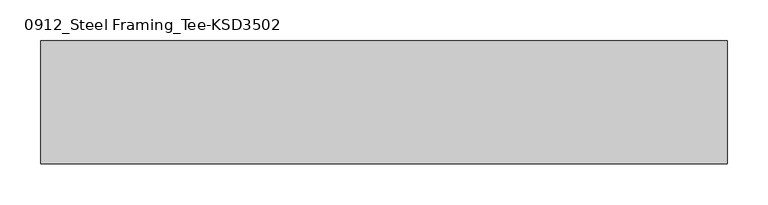
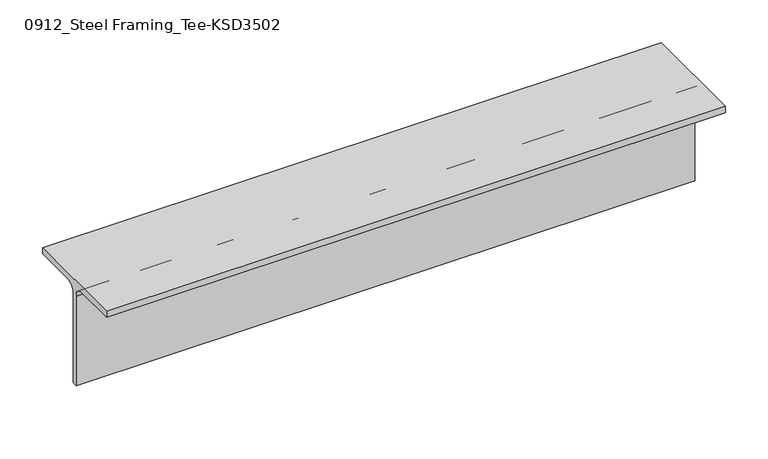
"""IFC4 building model written with IfcOpenShell, lengths in millimetres: member geometry, 0912_Steel Framing_Tee-KSD3502 : H_SB_ASB_CT-150x150x6.5x9."""

from ifc_helpers import new_model, si_unit, point, frame, frame_2d, origin, place, context, project, spatial, polyline, circle_curve, trimmed, segment, composite_curve, outline, extrude, source, transform, mapped, element, save


def member_0912_steel_framing_tee_ksd3502_cf34dda4(model_context):
    return source(origin(), model_context, "Body", "SweptSolid", [
        extrude(outline(composite_curve([segment(polyline([(-75.0, 75.0), (75.0, 75.0), (75.0, 66.0), (16.25, 66.0)]), True, "CONTINUOUS"), segment(trimmed(circle_curve(frame_2d((16.25, 53.0)), 13.0), [point((16.25, 66.0))], [point((3.25, 53.0))], True, "CARTESIAN"), True, "CONTINUOUS"), segment(polyline([(3.25, 53.0), (3.25, -75.0), (-3.25, -75.0), (-3.25, 53.0)]), True, "CONTINUOUS"), segment(trimmed(circle_curve(frame_2d((-16.25, 53.0)), 13.0), [point((-3.25, 53.0))], [point((-16.25, 66.0))], True, "CARTESIAN"), True, "CONTINUOUS"), segment(polyline([(-16.25, 66.0), (-75.0, 66.0), (-75.0, 75.0)]), True, "CONTINUOUS")], self_intersect=False)), frame((-500.0, 0.0, 0.0), z_axis=(1.0, 0.0, 0.0), x_axis=(0.0, 1.0, 0.0)), (0.0, 0.0, 1.0), 837.3),
    ])


if __name__ == "__main__":
    model = new_model("IFC4")
    model_context = context("Model", 3, world=origin())
    ifc_project = project(units=[si_unit("LENGTHUNIT", "METRE", prefix="MILLI")], contexts=[model_context])
    site = spatial("IfcSite", under=ifc_project)
    building = spatial("IfcBuilding", under=site)
    placement = place(None, origin())
    member_0912_steel_framing_tee_ksd3502_shape = member_0912_steel_framing_tee_ksd3502_cf34dda4(model_context)
    element("IfcMember", 1, ObjectType="0912_Steel Framing_Tee-KSD3502 : H_SB_ASB_CT-150x150x6.5x9", at=placement, inside=building, context=model_context, shape_type="MappedRepresentation", body=[
        mapped(member_0912_steel_framing_tee_ksd3502_shape, transform((0.0, 0.0, 0.0), x_axis=(1.0, 0.0, 0.0), y_axis=(0.0, 1.0, 0.0), z_axis=(0.0, 0.0, 1.0))),
    ])
    save(model, "model.ifc")

# Revit data of these elements
# Type "0912_Steel Framing_Tee-KSD3502 : H_SB_ASB_CT-150x150x6.5x9"
#   H_WM Code_1 = "S01AA003-00001 | Main Steel Structure Fabrication Work | Shelter/Building | Light Steel - Standard (30KG/M>Weight) | Material: (   )"
#   H_WM Code_2 = "S03AA029-00001 | Main Steel Structure Erection Work | Shelter/Building | Light Steel (30KG/M>Weight) | Material: (   )"
#   H_WM Code_3 = "S01AA010-00001 | Main Steel Structure Fabrication Work | Shelter/Building | Steel Painting/Coating | for Non-Fireproofed Steel Surface, Surface Preparation, Primer, Second & Final Coat | Material: (   )"
#   H_Q'ty Cal Type Tag = "SB-Q2"
#   Width = 15.0 cm
#   Web Thickness = 0.65 cm
#   Web Fillet = 1.3 cm
#   Section Area = 23.39 cm²
#   Perimeter = 0.60 m²/m
#   Nominal Weight = 18.40 kgf/m
#   Height = 15.0 cm
#   Flange Thickness = 0.9 cm
#   Centroid Vertical = 7.5 cm
#   Centroid Horizontal = 7.5 cm
#   Length [instance default] = 1.5000 m
#   Structural Material [instance default] = Steel, 45-345
#   Warping Constant = (empty or 0)
#   Torsional Moment of Inertia = 0
#   Section Name Key = ""
#   Plastic Modulus weak axis = 0
#   Plastic Modulus strong axis = 0
#   Moment of Inertia weak axis = 0
#   Moment of Inertia strong axis = 0
#   Elastic Modulus weak axis = 0
#   Elastic Modulus strong axis = 0
#   Bolt Spacing = 0
#   Assembly Code = ""
# Element 1 (IfcMember, "0912_Steel Framing_Tee-KSD3502 : H_SB_ASB_CT-150x150x6.5x9")
#   Structural Material = none
# Materials
#   "Steel, 45-345": class "Metal", colour RGB 189 187 185, transparency 0, Description = "Steel 345 MPa", Cost = 0
